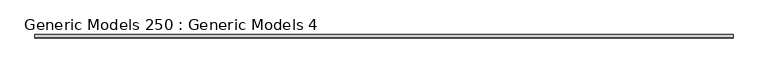
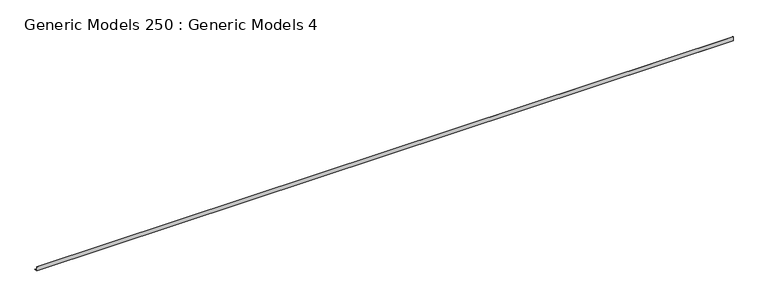
"""IFC4 building model written with IfcOpenShell, lengths in millimetres: proxy geometry, Generic Models 250 : Generic Models 4."""

from ifc_helpers import new_model, si_unit, frame, origin, place, context, project, spatial, polyline, outline, extrude, source, transform, mapped, element, save


def generic_models_250_generic_models_4_2e5e3241(model_context):
    return source(origin(), model_context, "Body", "SweptSolid", [
        extrude(outline(polyline([(11501.23061, 126904.4187), (11588.8621643, 126904.4187), (11588.8621643, 126903.62495), (11500.43686, 126903.62495), (11500.43686, 127018.9526629), (11501.23061, 127018.9526629), (11501.23061, 126904.4187)])), frame((-10234.5171316, 0.0, 0.0), z_axis=(1.0, 0.0, 0.0), x_axis=(0.0, 1.0, 0.0)), (0.0, 0.0, 1.0), 18643.6),
    ])


if __name__ == "__main__":
    model = new_model("IFC4")
    model_context = context("Model", 3, world=origin())
    ifc_project = project(units=[si_unit("LENGTHUNIT", "METRE", prefix="MILLI")], contexts=[model_context])
    site = spatial("IfcSite", under=ifc_project)
    building = spatial("IfcBuilding", under=site)
    placement = place(None, origin())
    generic_models_250_generic_models_4_shape = generic_models_250_generic_models_4_2e5e3241(model_context)
    element("IfcBuildingElementProxy", 1, Name="Generic Models 250 : Generic Models 4", ObjectType="Generic Models 250 : Generic Models 4", at=placement, inside=building, context=model_context, shape_type="MappedRepresentation", body=[
        mapped(generic_models_250_generic_models_4_shape, transform((0.0, 0.0, 0.0), x_axis=(1.0, 0.0, 0.0), y_axis=(0.0, 1.0, 0.0), z_axis=(0.0, 0.0, 1.0))),
    ])
    save(model, "model.ifc")

# Revit data of these elements
# Element 1 (IfcBuildingElementProxy, "Generic Models 250 : Generic Models 4")
#   Materials on its faces: "_16 GA. COPPER \"L\" FLASHING - (6\" HORZ. LEG - 4\" VERT. LEG)"
# Materials
#   "_16 GA. COPPER \"L\" FLASHING - (6\" HORZ. LEG - 4\" VERT. LEG)": class "Generic", colour RGB 156 184 169, transparency 0, Cost = 0
